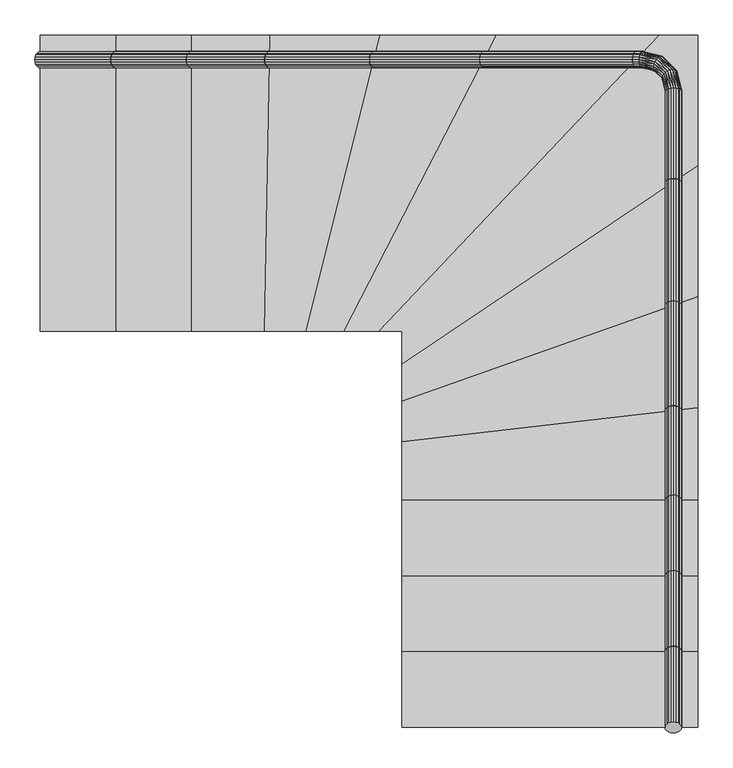
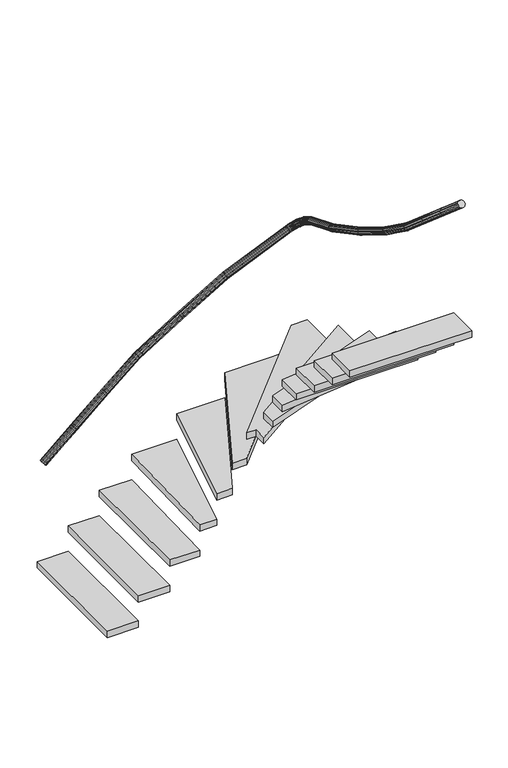
"""IFC4 building model written with IfcOpenShell, lengths in millimetres: stair geometry, 0_3d_modell."""

from ifc_helpers import new_model, si_unit, frame, origin, origin_with_axes, place, context, project, spatial, polyline, outline, extrude, faceted_brep, source, transform, mapped, element, save


def stair_c236abdd(model_context):
    return source(origin(), model_context, "Body", "SolidModel", [
        extrude(outline(polyline([(1049.2205336, 2121.5036957), (1403.2627923, 2121.5036957), (939.4821841, 1221.5036957), (824.5831846, 1221.5036957), (1049.2205336, 2121.5036957)])), frame((0.0, 0.0, 794.2857143), z_axis=(0.0, 0.0, 1.0), x_axis=(1.0, 0.0, 0.0)), (0.0, 0.0, 1.0), 50.0),
        faceted_brep([(1830.8955374, 2022.7272828, 2053.6142572), (1827.811235, 2021.5036957, 2060.987808), (1824.7269327, 2022.7272828, 2068.3613589), (1821.9445433, 2026.2782709, 2075.0131352), (1819.7364266, 2031.8090644, 2080.2920148), (1818.3187285, 2038.7782709, 2083.6812642), (1817.830223, 2046.5036957, 2084.8491199), (1818.3187285, 2054.2291206, 2083.6812642), (1819.7364266, 2061.198327, 2080.2920148), (1821.9445433, 2066.7291206, 2075.0131352), (1824.7269327, 2070.2801086, 2068.3613589), (1827.811235, 2071.5036957, 2060.987808), (1830.8955374, 2070.2801086, 2053.6142572), (1833.6779267, 2066.7291206, 2046.9624808), (1835.8860434, 2061.198327, 2041.6836012), (1837.3037416, 2054.2291206, 2038.2943519), (1837.7922471, 2046.5036957, 2037.1264962), (1837.3037416, 2038.7782709, 2038.2943519), (1835.8860434, 2031.8090644, 2041.6836012), (1833.6779267, 2026.2782709, 2046.9624808), (1918.1254462, 1677.2481385, 2266.8075559), (1916.9018591, 1673.856869, 2259.5592366), (1918.1254462, 1670.4655995, 2252.3109173), (1921.6764343, 1667.4062911, 2245.772114), (1927.2072278, 1664.9784102, 2240.5828904), (1934.1764343, 1663.4196147, 2237.2512037), (1941.9018591, 1662.8824904, 2236.1031827), (1949.627284, 1663.4196147, 2237.2512037), (1956.5964904, 1664.9784102, 2240.5828904), (1962.127284, 1667.4062911, 2245.772114), (1965.678272, 1670.4655995, 2252.3109173), (1966.9018591, 1673.856869, 2259.5592366), (1965.678272, 1677.2481385, 2266.8075559), (1962.127284, 1680.3074469, 2273.3463592), (1956.5964904, 1682.7353278, 2278.5355829), (1949.627284, 1684.2941233, 2281.8672695), (1941.9018591, 1684.8312476, 2283.0152905), (1934.1764343, 1684.2941233, 2281.8672695), (1927.2072278, 1682.7353278, 2278.5355829), (1921.6764343, 1680.3074469, 2273.3463592), (1846.1118218, 2021.5036957, 2068.4537913), (1843.0928107, 2022.7272828, 2075.8539787), (1840.3693214, 2026.2782709, 2082.5297841), (1838.2079481, 2031.8090644, 2087.8277333), (1836.820261, 2038.7782709, 2091.2292261), (1836.3420966, 2046.5036957, 2092.4013006), (1836.820261, 2054.2291206, 2091.2292261), (1838.2079481, 2061.198327, 2087.8277333), (1840.3693214, 2066.7291206, 2082.5297841), (1843.0928107, 2070.2801086, 2075.8539787), (1846.1118218, 2071.5036957, 2068.4537913), (1849.1308329, 2070.2801086, 2061.053604), (1851.8543222, 2066.7291206, 2054.3777985), (1854.0156955, 2061.198327, 2049.0798493), (1855.4033826, 2054.2291206, 2045.6783565), (1855.881547, 2046.5036957, 2044.506282), (1855.4033826, 2038.7782709, 2045.6783565), (1854.0156955, 2031.8090644, 2049.0798493), (1851.8543222, 2026.2782709, 2054.3777985), (1849.1308329, 2022.7272828, 2061.053604), (1884.7017207, 2012.6032946, 2093.9682441), (1881.8914919, 2015.5333905, 2100.9604911), (1880.5298735, 2020.3241085, 2107.2682883), (1880.7501499, 2026.5064996, 2112.2741844), (1882.5307592, 2033.4753883, 2115.4881676), (1885.6974028, 2040.5486112, 2116.5956307), (1889.9401076, 2047.0337921, 2115.4881676), (1894.8435681, 2052.2961161, 2112.2741844), (1899.9277994, 2055.8204705, 2107.2682883), (1904.6951215, 2057.2618667, 2100.9604911), (1908.6788758, 2056.4792109, 2093.9682441), (1911.4891045, 2053.549115, 2086.9759971), (1912.850723, 2048.758397, 2080.6681999), (1912.6304465, 2042.5760059, 2075.6623037), (1910.8498373, 2035.6071172, 2072.4483206), (1907.6831937, 2028.5338943, 2071.3408574), (1903.4404889, 2022.0487134, 2072.4483206), (1898.5370284, 2016.7863894, 2075.6623037), (1893.4527971, 2013.262035, 2080.6681999), (1888.685475, 2011.8206388, 2086.9759971), (1908.001458, 1989.3035573, 2121.0971401), (1907.2188022, 1993.2873116, 2128.0893871), (1908.6601984, 1998.0546337, 2134.3971843), (1912.1845528, 2003.138865, 2139.4030804), (1917.4468768, 2008.0423255, 2142.6170636), (1923.9320577, 2012.2850303, 2143.7245267), (1931.0052806, 2015.4516739, 2142.6170636), (1937.9741693, 2017.2322831, 2139.4030804), (1944.1565604, 2017.4525596, 2134.3971843), (1948.9472784, 2016.0909411, 2128.0893871), (1951.8773743, 2013.2807124, 2121.0971401), (1952.6600301, 2009.2969581, 2114.1048931), (1951.2186339, 2004.529636, 2107.7970959), (1947.6942795, 1999.4454047, 2102.7911997), (1942.4319555, 1994.5419442, 2099.5772166), (1935.9467746, 1990.2992394, 2098.4697534), (1928.8735517, 1987.1325958, 2099.5772166), (1921.904663, 1985.3519865, 2102.7911997), (1915.7222719, 1985.1317101, 2107.7970959), (1910.9315539, 1986.4933285, 2114.1048931), (1916.9018591, 1950.7136584, 2146.6115929), (1918.1254462, 1953.7326696, 2154.0117802), (1921.6764343, 1956.4561588, 2160.6875857), (1927.2072278, 1958.6175321, 2165.9855349), (1934.1764343, 1960.0052192, 2169.3870277), (1941.9018591, 1960.4833836, 2170.5591022), (1949.627284, 1960.0052192, 2169.3870277), (1956.5964904, 1958.6175321, 2165.9855349), (1962.127284, 1956.4561588, 2160.6875857), (1965.678272, 1953.7326696, 2154.0117802), (1966.9018591, 1950.7136584, 2146.6115929), (1965.678272, 1947.6946473, 2139.2114055), (1962.127284, 1944.971158, 2132.5356001), (1956.5964904, 1942.8097847, 2127.2376509), (1949.627284, 1941.4220976, 2123.8361581), (1941.9018591, 1940.9439332, 2122.6640835), (1934.1764343, 1941.4220976, 2123.8361581), (1927.2072278, 1942.8097847, 2127.2376509), (1921.6764343, 1944.971158, 2132.5356001), (1918.1254462, 1947.6946473, 2139.2114055)], [[[0, 1, 2, 3, 4, 5, 6, 7, 8, 9, 10, 11, 12, 13, 14, 15, 16, 17, 18, 19]], [[20, 21, 22, 23, 24, 25, 26, 27, 28, 29, 30, 31, 32, 33, 34, 35, 36, 37, 38, 39]], [[2, 1, 40, 41]], [[3, 2, 41, 42]], [[4, 3, 42, 43]], [[5, 4, 43, 44]], [[6, 5, 44, 45]], [[7, 6, 45, 46]], [[8, 7, 46, 47]], [[9, 8, 47, 48]], [[10, 9, 48, 49]], [[11, 10, 49, 50]], [[12, 11, 50, 51]], [[13, 12, 51, 52]], [[14, 13, 52, 53]], [[15, 14, 53, 54]], [[16, 15, 54, 55]], [[17, 16, 55, 56]], [[18, 17, 56, 57]], [[19, 18, 57, 58]], [[0, 19, 58, 59]], [[1, 0, 59, 40]], [[41, 40, 60]], [[61, 41, 60]], [[42, 41, 61]], [[62, 42, 61]], [[43, 42, 62]], [[63, 43, 62]], [[44, 43, 63]], [[64, 44, 63]], [[45, 44, 64]], [[65, 45, 64]], [[46, 45, 65]], [[66, 46, 65]], [[47, 46, 66]], [[67, 47, 66]], [[48, 47, 67]], [[68, 48, 67]], [[49, 48, 68]], [[69, 49, 68]], [[50, 49, 69]], [[70, 50, 69]], [[51, 50, 70]], [[71, 51, 70]], [[52, 51, 71]], [[72, 52, 71]], [[53, 52, 72]], [[73, 53, 72]], [[54, 53, 73]], [[74, 54, 73]], [[55, 54, 74]], [[75, 55, 74]], [[56, 55, 75]], [[76, 56, 75]], [[57, 56, 76]], [[77, 57, 76]], [[58, 57, 77]], [[78, 58, 77]], [[59, 58, 78]], [[79, 59, 78]], [[40, 59, 79]], [[60, 40, 79]], [[61, 60, 80]], [[81, 61, 80]], [[62, 61, 81]], [[82, 62, 81]], [[63, 62, 82]], [[83, 63, 82]], [[64, 63, 83]], [[84, 64, 83]], [[65, 64, 84]], [[85, 65, 84]], [[66, 65, 85]], [[86, 66, 85]], [[67, 66, 86]], [[87, 67, 86]], [[68, 67, 87]], [[88, 68, 87]], [[69, 68, 88]], [[89, 69, 88]], [[70, 69, 89]], [[90, 70, 89]], [[71, 70, 90]], [[91, 71, 90]], [[72, 71, 91]], [[92, 72, 91]], [[73, 72, 92]], [[93, 73, 92]], [[74, 73, 93]], [[94, 74, 93]], [[75, 74, 94]], [[95, 75, 94]], [[76, 75, 95]], [[96, 76, 95]], [[77, 76, 96]], [[97, 77, 96]], [[78, 77, 97]], [[98, 78, 97]], [[79, 78, 98]], [[99, 79, 98]], [[60, 79, 99]], [[80, 60, 99]], [[81, 80, 100]], [[101, 81, 100]], [[82, 81, 101]], [[102, 82, 101]], [[83, 82, 102]], [[103, 83, 102]], [[84, 83, 103]], [[104, 84, 103]], [[85, 84, 104]], [[105, 85, 104]], [[86, 85, 105]], [[106, 86, 105]], [[87, 86, 106]], [[107, 87, 106]], [[88, 87, 107]], [[108, 88, 107]], [[89, 88, 108]], [[109, 89, 108]], [[90, 89, 109]], [[110, 90, 109]], [[91, 90, 110]], [[111, 91, 110]], [[92, 91, 111]], [[112, 92, 111]], [[93, 92, 112]], [[113, 93, 112]], [[94, 93, 113]], [[114, 94, 113]], [[95, 94, 114]], [[115, 95, 114]], [[96, 95, 115]], [[116, 96, 115]], [[97, 96, 116]], [[117, 97, 116]], [[98, 97, 117]], [[118, 98, 117]], [[99, 98, 118]], [[119, 99, 118]], [[80, 99, 119]], [[100, 80, 119]], [[101, 100, 21, 20]], [[102, 101, 20, 39]], [[103, 102, 39, 38]], [[104, 103, 38, 37]], [[105, 104, 37, 36]], [[106, 105, 36, 35]], [[107, 106, 35, 34]], [[108, 107, 34, 33]], [[109, 108, 33, 32]], [[110, 109, 32, 31]], [[111, 110, 31, 30]], [[112, 111, 30, 29]], [[113, 112, 29, 28]], [[114, 113, 28, 27]], [[115, 114, 27, 26]], [[116, 115, 26, 25]], [[117, 116, 25, 24]], [[118, 117, 24, 23]], [[119, 118, 23, 22]], [[100, 119, 22, 21]]]),
        extrude(outline(polyline([(2016.9018591, 1724.0707938), (2016.9018591, 1326.2140709), (1116.9018591, 1007.5896473), (1116.9018591, 1121.5036957), (2016.9018591, 1724.0707938)])), frame((0.0, 0.0, 1390.0), z_axis=(0.0, 0.0, 1.0), x_axis=(1.0, 0.0, 0.0)), (0.0, 0.0, 1.0), 50.0),
        extrude(outline(polyline([(1.2235871, -7.9923214), (0.0, 0.0), (1.2235871, 7.9923214), (4.7745752, 15.2022986), (10.3053687, 20.924169), (17.2745752, 24.5978359), (25.0, 25.8636953), (32.7254249, 24.5978359), (39.6946313, 20.924169), (45.2254249, 15.2022986), (48.7764129, 7.9923214), (50.0, 0.0), (48.7764129, -7.9923214), (45.2254249, -15.2022986), (39.6946313, -20.9241691), (32.7254249, -24.5978359), (25.0, -25.8636953), (17.2745752, -24.5978359), (10.3053687, -20.9241691), (4.7745752, -15.2022986), (1.2235871, -7.9923214)])), frame((16.9018591, 2021.5036957, 869.5592366), z_axis=(0.756928710285757, 0.0, 0.6534974579484916), x_axis=(0.0, 1.0, 0.0)), (0.0, 0.0, 1.0), 303.8595272),
        extrude(outline(polyline([(246.9018591, 2121.5036957), (476.9018591, 2121.5036957), (476.9018591, 1221.5036957), (246.9018591, 1221.5036957), (246.9018591, 2121.5036957)])), frame((0.0, 0.0, 198.5714286), z_axis=(0.0, 0.0, 1.0), x_axis=(1.0, 0.0, 0.0)), (0.0, 0.0, 1.0), 50.0),
        extrude(outline(polyline([(2016.9018591, 476.9018591), (2016.9018591, 246.9018591), (1116.9018591, 246.9018591), (1116.9018591, 476.9018591), (2016.9018591, 476.9018591)])), frame((0.0, 0.0, 2184.2857143), z_axis=(0.0, 0.0, 1.0), x_axis=(1.0, 0.0, 0.0)), (0.0, 0.0, 1.0), 50.0),
        extrude(outline(polyline([(2016.9018591, 1326.2140709), (2016.9018591, 988.8933271), (1116.9018591, 884.9103911), (1116.9018591, 1007.5896473), (2016.9018591, 1326.2140709)])), frame((0.0, 0.0, 1588.5714286), z_axis=(0.0, 0.0, 1.0), x_axis=(1.0, 0.0, 0.0)), (0.0, 0.0, 1.0), 50.0),
        faceted_brep([(1918.1254462, 1295.6744399, 2451.1987943), (1916.9018591, 1299.6620356, 2458.1306652), (1918.1254462, 1303.6496314, 2465.062536), (1921.6764343, 1307.2468935, 2471.3158671), (1927.2072278, 1310.1016969, 2476.2785387), (1934.1764343, 1311.9345935, 2479.46477), (1941.9018591, 1312.5661666, 2480.5626705), (1949.627284, 1311.9345935, 2479.46477), (1956.5964904, 1310.1016969, 2476.2785387), (1962.127284, 1307.2468935, 2471.3158671), (1965.678272, 1303.6496314, 2465.062536), (1966.9018591, 1299.6620356, 2458.1306652), (1965.678272, 1295.6744399, 2451.1987943), (1962.127284, 1292.0771778, 2444.9454632), (1956.5964904, 1289.2223744, 2439.9827916), (1949.627284, 1287.3894778, 2436.7965603), (1941.9018591, 1286.7579047, 2435.6986598), (1934.1764343, 1287.3894778, 2436.7965603), (1927.2072278, 1289.2223744, 2439.9827916), (1921.6764343, 1292.0771778, 2444.9454632), (1918.1254462, 984.692421, 2663.3376045), (1916.9018591, 980.2280824, 2656.7020937), (1918.1254462, 975.7637439, 2650.066583), (1921.6764343, 971.7364059, 2644.0806023), (1927.2072278, 968.5402924, 2639.3301012), (1934.1764343, 966.4882612, 2636.2800917), (1941.9018591, 965.7811794, 2635.22913), (1949.627284, 966.4882612, 2636.2800917), (1956.5964904, 968.5402924, 2639.3301012), (1962.127284, 971.7364059, 2644.0806023), (1965.678272, 975.7637439, 2650.066583), (1966.9018591, 980.2280824, 2656.7020937), (1965.678272, 984.692421, 2663.3376045), (1962.127284, 988.719759, 2669.3235852), (1956.5964904, 991.9158725, 2674.0740863), (1949.627284, 993.9679037, 2677.1240958), (1941.9018591, 994.6749855, 2678.1750575), (1934.1764343, 993.9679037, 2677.1240958), (1927.2072278, 991.9158725, 2674.0740863), (1921.6764343, 988.719759, 2669.3235852)], [[[0, 1, 2, 3, 4, 5, 6, 7, 8, 9, 10, 11, 12, 13, 14, 15, 16, 17, 18, 19]], [[20, 21, 22, 23, 24, 25, 26, 27, 28, 29, 30, 31, 32, 33, 34, 35, 36, 37, 38, 39]], [[2, 1, 21, 20]], [[3, 2, 20, 39]], [[4, 3, 39, 38]], [[5, 4, 38, 37]], [[6, 5, 37, 36]], [[7, 6, 36, 35]], [[8, 7, 35, 34]], [[9, 8, 34, 33]], [[10, 9, 33, 32]], [[11, 10, 32, 31]], [[12, 11, 31, 30]], [[13, 12, 30, 29]], [[14, 13, 29, 28]], [[15, 14, 28, 27]], [[16, 15, 27, 26]], [[17, 16, 26, 25]], [[18, 17, 25, 24]], [[19, 18, 24, 23]], [[0, 19, 23, 22]], [[1, 0, 22, 21]]]),
        extrude(outline(polyline([(16.9018591, 2121.5036957), (246.9018591, 2121.5036957), (246.9018591, 1221.5036957), (16.9018591, 1221.5036957), (16.9018591, 2121.5036957)])), origin_with_axes(), (0.0, 0.0, 1.0), 50.0),
        faceted_brep([(482.0819027, 2022.7272828, 1260.6154227), (476.9018591, 2021.5036957, 1266.7020937), (471.7218155, 2022.7272828, 1272.7887648), (467.0488307, 2026.2782709, 1278.2796301), (463.340329, 2031.8090644, 1282.6372054), (460.9593243, 2038.7782709, 1285.434941), (460.138886, 2046.5036957, 1286.398975), (460.9593243, 2054.2291206, 1285.434941), (463.340329, 2061.198327, 1282.6372054), (467.0488307, 2066.7291206, 1278.2796301), (471.7218155, 2070.2801086, 1272.7887648), (476.9018591, 2071.5036957, 1266.7020937), (482.0819027, 2070.2801086, 1260.6154227), (486.7548875, 2066.7291206, 1255.1245574), (490.4633893, 2061.198327, 1250.7669821), (492.844394, 2054.2291206, 1247.9692465), (493.6648323, 2046.5036957, 1247.0052125), (492.844394, 2038.7782709, 1247.9692465), (490.4633893, 2031.8090644, 1250.7669821), (486.7548875, 2026.2782709, 1255.1245574), (708.8971261, 2022.7272828, 1471.7522459), (713.6098217, 2021.5036957, 1465.2735223), (718.3225173, 2022.7272828, 1458.7947987), (722.5739015, 2026.2782709, 1452.9502578), (725.947819, 2031.8090644, 1448.3120038), (728.1140074, 2038.7782709, 1445.3340614), (728.8604251, 2046.5036957, 1444.3079324), (728.1140074, 2054.2291206, 1445.3340614), (725.947819, 2061.198327, 1448.3120038), (722.5739015, 2066.7291206, 1452.9502578), (718.3225173, 2070.2801086, 1458.7947987), (713.6098217, 2071.5036957, 1465.2735223), (708.8971261, 2070.2801086, 1471.7522459), (704.645742, 2066.7291206, 1477.5967869), (701.2718245, 2061.198327, 1482.2350408), (699.1056361, 2054.2291206, 1485.2129832), (698.3592184, 2046.5036957, 1486.2391122), (699.1056361, 2038.7782709, 1485.2129832), (701.2718245, 2031.8090644, 1482.2350408), (704.645742, 2026.2782709, 1477.5967869)], [[[0, 1, 2, 3, 4, 5, 6, 7, 8, 9, 10, 11, 12, 13, 14, 15, 16, 17, 18, 19]], [[20, 21, 22, 23, 24, 25, 26, 27, 28, 29, 30, 31, 32, 33, 34, 35, 36, 37, 38, 39]], [[2, 1, 21, 20]], [[3, 2, 20, 39]], [[4, 3, 39, 38]], [[5, 4, 38, 37]], [[6, 5, 37, 36]], [[7, 6, 36, 35]], [[8, 7, 35, 34]], [[9, 8, 34, 33]], [[10, 9, 33, 32]], [[11, 10, 32, 31]], [[12, 11, 31, 30]], [[13, 12, 30, 29]], [[14, 13, 29, 28]], [[15, 14, 28, 27]], [[16, 15, 27, 26]], [[17, 16, 26, 25]], [[18, 17, 25, 24]], [[19, 18, 24, 23]], [[0, 19, 23, 22]], [[1, 0, 22, 21]]]),
        extrude(outline(polyline([(1403.2627923, 2121.5036957), (1898.8029965, 2121.5036957), (1046.9018591, 1221.5036957), (939.4821841, 1221.5036957), (1403.2627923, 2121.5036957)])), frame((0.0, 0.0, 992.8571429), z_axis=(0.0, 0.0, 1.0), x_axis=(1.0, 0.0, 0.0)), (0.0, 0.0, 1.0), 50.0),
        extrude(outline(polyline([(2016.9018591, 246.9018591), (2016.9018591, 16.9018591), (1116.9018591, 16.9018591), (1116.9018591, 246.9018591), (2016.9018591, 246.9018591)])), frame((0.0, 0.0, 2382.8571429), z_axis=(0.0, 0.0, 1.0), x_axis=(1.0, 0.0, 0.0)), (0.0, 0.0, 1.0), 50.0),
        faceted_brep([(252.1248208, 2022.7272828, 1062.0810477), (246.9018591, 2021.5036957, 1068.1306652), (241.6788974, 2022.7272828, 1074.1802827), (236.9671956, 2026.2782709, 1079.6377215), (233.2279679, 2031.8090644, 1083.9687694), (230.8272359, 2038.7782709, 1086.7494734), (230.0, 2046.5036957, 1087.7076387), (230.8272359, 2054.2291206, 1086.7494734), (233.2279679, 2061.198327, 1083.9687694), (236.9671956, 2066.7291206, 1079.6377215), (241.6788974, 2070.2801086, 1074.1802827), (246.9018591, 2071.5036957, 1068.1306652), (252.1248208, 2070.2801086, 1062.0810477), (256.8365226, 2066.7291206, 1056.6236089), (260.5757504, 2061.198327, 1052.2925609), (262.9764824, 2054.2291206, 1049.511857), (263.8037182, 2046.5036957, 1048.5536917), (262.9764824, 2038.7782709, 1049.511857), (260.5757504, 2031.8090644, 1052.2925609), (256.8365226, 2026.2782709, 1056.6236089), (471.7218155, 2022.7272828, 1272.7887648), (476.9018591, 2021.5036957, 1266.7020937), (482.0819027, 2022.7272828, 1260.6154227), (486.7548875, 2026.2782709, 1255.1245574), (490.4633893, 2031.8090644, 1250.7669821), (492.844394, 2038.7782709, 1247.9692465), (493.6648323, 2046.5036957, 1247.0052125), (492.844394, 2054.2291206, 1247.9692465), (490.4633893, 2061.198327, 1250.7669821), (486.7548875, 2066.7291206, 1255.1245574), (482.0819027, 2070.2801086, 1260.6154227), (476.9018591, 2071.5036957, 1266.7020937), (471.7218155, 2070.2801086, 1272.7887648), (467.0488307, 2066.7291206, 1278.2796301), (463.340329, 2061.198327, 1282.6372054), (460.9593243, 2054.2291206, 1285.434941), (460.138886, 2046.5036957, 1286.398975), (460.9593243, 2038.7782709, 1285.434941), (463.340329, 2031.8090644, 1282.6372054), (467.0488307, 2026.2782709, 1278.2796301)], [[[0, 1, 2, 3, 4, 5, 6, 7, 8, 9, 10, 11, 12, 13, 14, 15, 16, 17, 18, 19]], [[20, 21, 22, 23, 24, 25, 26, 27, 28, 29, 30, 31, 32, 33, 34, 35, 36, 37, 38, 39]], [[2, 1, 21, 20]], [[3, 2, 20, 39]], [[4, 3, 39, 38]], [[5, 4, 38, 37]], [[6, 5, 37, 36]], [[7, 6, 36, 35]], [[8, 7, 35, 34]], [[9, 8, 34, 33]], [[10, 9, 33, 32]], [[11, 10, 32, 31]], [[12, 11, 31, 30]], [[13, 12, 30, 29]], [[14, 13, 29, 28]], [[15, 14, 28, 27]], [[16, 15, 27, 26]], [[17, 16, 26, 25]], [[18, 17, 25, 24]], [[19, 18, 24, 23]], [[0, 19, 23, 22]], [[1, 0, 22, 21]]]),
        extrude(outline(polyline([(2016.9018591, 706.9018591), (2016.9018591, 476.9018591), (1116.9018591, 476.9018591), (1116.9018591, 706.9018591), (2016.9018591, 706.9018591)])), frame((0.0, 0.0, 1985.7142857), z_axis=(0.0, 0.0, 1.0), x_axis=(1.0, 0.0, 0.0)), (0.0, 0.0, 1.0), 50.0),
        extrude(outline(polyline([(1898.8029965, 2121.5036957), (2016.9018591, 2121.5036957), (2016.9018591, 1724.0707938), (1116.9018591, 1121.5036957), (1116.9018591, 1221.5036957), (1046.9018591, 1221.5036957), (1898.8029965, 2121.5036957)])), frame((0.0, 0.0, 1191.4285714), z_axis=(0.0, 0.0, 1.0), x_axis=(1.0, 0.0, 0.0)), (0.0, 0.0, 1.0), 50.0),
        extrude(outline(polyline([(1.2235871, -7.9923214), (0.0, 0.0), (1.2235871, 7.9923214), (4.7745752, 15.2022986), (10.3053687, 20.9241691), (17.2745752, 24.5978359), (25.0, 25.8636953), (32.7254249, 24.5978359), (39.6946313, 20.9241691), (45.2254249, 15.2022986), (48.7764129, 7.9923214), (50.0, 0.0), (48.7764129, -7.9923214), (45.2254249, -15.2022986), (39.6946313, -20.924169), (32.7254249, -24.5978359), (25.0, -25.8636953), (17.2745752, -24.5978359), (10.3053687, -20.924169), (4.7745752, -15.2022986), (1.2235871, -7.9923214)])), frame((1916.9018591, 476.9018591, 3053.8449509), z_axis=(0.0, -0.7569287102856931, 0.6534974579485656), x_axis=(1.0, 0.0, 0.0)), (0.0, 0.0, 1.0), 303.8595272),
        faceted_brep([(1918.1254462, 701.932844, 2849.004659), (1916.9018591, 706.9018591, 2855.2735223), (1918.1254462, 711.8708742, 2861.5423857), (1921.6764343, 716.3534875, 2867.197609), (1927.2072278, 719.9109095, 2871.6856196), (1934.1764343, 722.194915, 2874.5670998), (1941.9018591, 722.9819297, 2875.5599903), (1949.627284, 722.194915, 2874.5670998), (1956.5964904, 719.9109095, 2871.6856196), (1962.127284, 716.3534875, 2867.197609), (1965.678272, 711.8708742, 2861.5423857), (1966.9018591, 706.9018591, 2855.2735223), (1965.678272, 701.932844, 2849.004659), (1962.127284, 697.4502308, 2843.3494356), (1956.5964904, 693.8928087, 2838.861425), (1949.627284, 691.6088032, 2835.9799448), (1941.9018591, 690.8217885, 2834.9870544), (1934.1764343, 691.6088032, 2835.9799448), (1927.2072278, 693.8928087, 2838.861425), (1921.6764343, 697.4502308, 2843.3494356), (1918.1254462, 482.1248208, 3059.8945684), (1916.9018591, 476.9018591, 3053.8449509), (1918.1254462, 471.6788974, 3047.7953334), (1921.6764343, 466.9671956, 3042.3378946), (1927.2072278, 463.2279679, 3038.0068466), (1934.1764343, 460.8272359, 3035.2261427), (1941.9018591, 460.0, 3034.2679774), (1949.627284, 460.8272359, 3035.2261427), (1956.5964904, 463.2279679, 3038.0068466), (1962.127284, 466.9671956, 3042.3378946), (1965.678272, 471.6788974, 3047.7953334), (1966.9018591, 476.9018591, 3053.8449509), (1965.678272, 482.1248208, 3059.8945684), (1962.127284, 486.8365226, 3065.3520072), (1956.5964904, 490.5757504, 3069.6830552), (1949.627284, 492.9764824, 3072.4637591), (1941.9018591, 493.8037182, 3073.4219244), (1934.1764343, 492.9764824, 3072.4637591), (1927.2072278, 490.5757504, 3069.6830552), (1921.6764343, 486.8365226, 3065.3520072)], [[[0, 1, 2, 3, 4, 5, 6, 7, 8, 9, 10, 11, 12, 13, 14, 15, 16, 17, 18, 19]], [[20, 21, 22, 23, 24, 25, 26, 27, 28, 29, 30, 31, 32, 33, 34, 35, 36, 37, 38, 39]], [[2, 1, 21, 20]], [[3, 2, 20, 39]], [[4, 3, 39, 38]], [[5, 4, 38, 37]], [[6, 5, 37, 36]], [[7, 6, 36, 35]], [[8, 7, 35, 34]], [[9, 8, 34, 33]], [[10, 9, 33, 32]], [[11, 10, 32, 31]], [[12, 11, 31, 30]], [[13, 12, 30, 29]], [[14, 13, 29, 28]], [[15, 14, 28, 27]], [[16, 15, 27, 26]], [[17, 16, 26, 25]], [[18, 17, 25, 24]], [[19, 18, 24, 23]], [[0, 19, 23, 22]], [[1, 0, 22, 21]]]),
        faceted_brep([(1368.2462303, 2022.7272828, 1855.277549), (1364.6144083, 2021.5036957, 1862.4163795), (1360.9825862, 2022.7272828, 1869.5552099), (1357.7062723, 2026.2782709, 1875.9952419), (1355.1061748, 2031.8090644, 1881.1060802), (1353.4368094, 2038.7782709, 1884.3874404), (1352.8615853, 2046.5036957, 1885.51812), (1353.4368094, 2054.2291206, 1884.3874404), (1355.1061748, 2061.198327, 1881.1060802), (1357.7062723, 2066.7291206, 1875.9952419), (1360.9825862, 2070.2801086, 1869.5552099), (1364.6144083, 2071.5036957, 1862.4163795), (1368.2462303, 2070.2801086, 1855.277549), (1371.5225443, 2066.7291206, 1848.8375171), (1374.1226418, 2061.198327, 1843.7266788), (1375.7920071, 2054.2291206, 1840.4453186), (1376.3672312, 2046.5036957, 1839.3146389), (1375.7920071, 2038.7782709, 1840.4453186), (1374.1226418, 2031.8090644, 1843.7266788), (1371.5225443, 2026.2782709, 1848.8375171), (1824.7269327, 2022.7272828, 2068.3613589), (1827.811235, 2021.5036957, 2060.987808), (1830.8955374, 2022.7272828, 2053.6142572), (1833.6779267, 2026.2782709, 2046.9624808), (1835.8860434, 2031.8090644, 2041.6836012), (1837.3037416, 2038.7782709, 2038.2943519), (1837.7922471, 2046.5036957, 2037.1264962), (1837.3037416, 2054.2291206, 2038.2943519), (1835.8860434, 2061.198327, 2041.6836012), (1833.6779267, 2066.7291206, 2046.9624808), (1830.8955374, 2070.2801086, 2053.6142572), (1827.811235, 2071.5036957, 2060.987808), (1824.7269327, 2070.2801086, 2068.3613589), (1821.9445433, 2066.7291206, 2075.0131352), (1819.7364266, 2061.198327, 2080.2920148), (1818.3187285, 2054.2291206, 2083.6812642), (1817.830223, 2046.5036957, 2084.8491199), (1818.3187285, 2038.7782709, 2083.6812642), (1819.7364266, 2031.8090644, 2080.2920148), (1821.9445433, 2026.2782709, 2075.0131352)], [[[0, 1, 2, 3, 4, 5, 6, 7, 8, 9, 10, 11, 12, 13, 14, 15, 16, 17, 18, 19]], [[20, 21, 22, 23, 24, 25, 26, 27, 28, 29, 30, 31, 32, 33, 34, 35, 36, 37, 38, 39]], [[2, 1, 21, 20]], [[3, 2, 20, 39]], [[4, 3, 39, 38]], [[5, 4, 38, 37]], [[6, 5, 37, 36]], [[7, 6, 36, 35]], [[8, 7, 35, 34]], [[9, 8, 34, 33]], [[10, 9, 33, 32]], [[11, 10, 32, 31]], [[12, 11, 31, 30]], [[13, 12, 30, 29]], [[14, 13, 29, 28]], [[15, 14, 28, 27]], [[16, 15, 27, 26]], [[17, 16, 26, 25]], [[18, 17, 25, 24]], [[19, 18, 24, 23]], [[0, 19, 23, 22]], [[1, 0, 22, 21]]]),
        faceted_brep([(718.3225173, 2022.7272828, 1458.7947987), (713.6098217, 2021.5036957, 1465.2735223), (708.8971261, 2022.7272828, 1471.7522459), (704.645742, 2026.2782709, 1477.5967869), (701.2718245, 2031.8090644, 1482.2350408), (699.1056361, 2038.7782709, 1485.2129832), (698.3592184, 2046.5036957, 1486.2391122), (699.1056361, 2054.2291206, 1485.2129832), (701.2718245, 2061.198327, 1482.2350408), (704.645742, 2066.7291206, 1477.5967869), (708.8971261, 2070.2801086, 1471.7522459), (713.6098217, 2071.5036957, 1465.2735223), (718.3225173, 2070.2801086, 1458.7947987), (722.5739015, 2066.7291206, 1452.9502578), (725.947819, 2061.198327, 1448.3120038), (728.1140074, 2054.2291206, 1445.3340614), (728.8604251, 2046.5036957, 1444.3079324), (728.1140074, 2038.7782709, 1445.3340614), (725.947819, 2031.8090644, 1448.3120038), (722.5739015, 2026.2782709, 1452.9502578), (1026.3366143, 2022.7272828, 1670.6674124), (1030.5007545, 2021.5036957, 1663.8449509), (1034.6648948, 2022.7272828, 1657.0224894), (1038.42142, 2026.2782709, 1650.867858), (1041.4026152, 2031.8090644, 1645.9835149), (1043.3166604, 2038.7782709, 1642.8475735), (1043.9761954, 2046.5036957, 1641.7670018), (1043.3166604, 2054.2291206, 1642.8475735), (1041.4026152, 2061.198327, 1645.9835149), (1038.42142, 2066.7291206, 1650.867858), (1034.6648948, 2070.2801086, 1657.0224894), (1030.5007545, 2071.5036957, 1663.8449509), (1026.3366143, 2070.2801086, 1670.6674124), (1022.5800891, 2066.7291206, 1676.8220438), (1019.5988939, 2061.198327, 1681.7063869), (1017.6848487, 2054.2291206, 1684.8423282), (1017.0253137, 2046.5036957, 1685.9229), (1017.6848487, 2038.7782709, 1684.8423282), (1019.5988939, 2031.8090644, 1681.7063869), (1022.5800891, 2026.2782709, 1676.8220438)], [[[0, 1, 2, 3, 4, 5, 6, 7, 8, 9, 10, 11, 12, 13, 14, 15, 16, 17, 18, 19]], [[20, 21, 22, 23, 24, 25, 26, 27, 28, 29, 30, 31, 32, 33, 34, 35, 36, 37, 38, 39]], [[2, 1, 21, 20]], [[3, 2, 20, 39]], [[4, 3, 39, 38]], [[5, 4, 38, 37]], [[6, 5, 37, 36]], [[7, 6, 36, 35]], [[8, 7, 35, 34]], [[9, 8, 34, 33]], [[10, 9, 33, 32]], [[11, 10, 32, 31]], [[12, 11, 31, 30]], [[13, 12, 30, 29]], [[14, 13, 29, 28]], [[15, 14, 28, 27]], [[16, 15, 27, 26]], [[17, 16, 26, 25]], [[18, 17, 25, 24]], [[19, 18, 24, 23]], [[0, 19, 23, 22]], [[1, 0, 22, 21]]]),
        extrude(outline(polyline([(476.9018591, 2121.5036957), (714.9514143, 2121.5036957), (698.852304, 1221.5036957), (476.9018591, 1221.5036957), (476.9018591, 2121.5036957)])), frame((0.0, 0.0, 397.1428571), z_axis=(0.0, 0.0, 1.0), x_axis=(1.0, 0.0, 0.0)), (0.0, 0.0, 1.0), 50.0),
        extrude(outline(polyline([(2016.9018591, 988.8933271), (2016.9018591, 706.9018591), (1116.9018591, 706.9018591), (1116.9018591, 884.9103911), (2016.9018591, 988.8933271)])), frame((0.0, 0.0, 1787.1428571), z_axis=(0.0, 0.0, 1.0), x_axis=(1.0, 0.0, 0.0)), (0.0, 0.0, 1.0), 50.0),
        faceted_brep([(1034.6648948, 2022.7272828, 1657.0224894), (1030.5007545, 2021.5036957, 1663.8449509), (1026.3366143, 2022.7272828, 1670.6674124), (1022.5800891, 2026.2782709, 1676.8220438), (1019.5988939, 2031.8090644, 1681.7063869), (1017.6848487, 2038.7782709, 1684.8423282), (1017.0253137, 2046.5036957, 1685.9229), (1017.6848487, 2054.2291206, 1684.8423282), (1019.5988939, 2061.198327, 1681.7063869), (1022.5800891, 2066.7291206, 1676.8220438), (1026.3366143, 2070.2801086, 1670.6674124), (1030.5007545, 2071.5036957, 1663.8449509), (1034.6648948, 2070.2801086, 1657.0224894), (1038.42142, 2066.7291206, 1650.867858), (1041.4026152, 2061.198327, 1645.9835149), (1043.3166604, 2054.2291206, 1642.8475735), (1043.9761954, 2046.5036957, 1641.7670018), (1043.3166604, 2038.7782709, 1642.8475735), (1041.4026152, 2031.8090644, 1645.9835149), (1038.42142, 2026.2782709, 1650.867858), (1360.9825862, 2022.7272828, 1869.5552099), (1364.6144083, 2021.5036957, 1862.4163795), (1368.2462303, 2022.7272828, 1855.277549), (1371.5225443, 2026.2782709, 1848.8375171), (1374.1226418, 2031.8090644, 1843.7266788), (1375.7920071, 2038.7782709, 1840.4453186), (1376.3672312, 2046.5036957, 1839.3146389), (1375.7920071, 2054.2291206, 1840.4453186), (1374.1226418, 2061.198327, 1843.7266788), (1371.5225443, 2066.7291206, 1848.8375171), (1368.2462303, 2070.2801086, 1855.277549), (1364.6144083, 2071.5036957, 1862.4163795), (1360.9825862, 2070.2801086, 1869.5552099), (1357.7062723, 2066.7291206, 1875.9952419), (1355.1061748, 2061.198327, 1881.1060802), (1353.4368094, 2054.2291206, 1884.3874404), (1352.8615853, 2046.5036957, 1885.51812), (1353.4368094, 2038.7782709, 1884.3874404), (1355.1061748, 2031.8090644, 1881.1060802), (1357.7062723, 2026.2782709, 1875.9952419)], [[[0, 1, 2, 3, 4, 5, 6, 7, 8, 9, 10, 11, 12, 13, 14, 15, 16, 17, 18, 19]], [[20, 21, 22, 23, 24, 25, 26, 27, 28, 29, 30, 31, 32, 33, 34, 35, 36, 37, 38, 39]], [[2, 1, 21, 20]], [[3, 2, 20, 39]], [[4, 3, 39, 38]], [[5, 4, 38, 37]], [[6, 5, 37, 36]], [[7, 6, 36, 35]], [[8, 7, 35, 34]], [[9, 8, 34, 33]], [[10, 9, 33, 32]], [[11, 10, 32, 31]], [[12, 11, 31, 30]], [[13, 12, 30, 29]], [[14, 13, 29, 28]], [[15, 14, 28, 27]], [[16, 15, 27, 26]], [[17, 16, 26, 25]], [[18, 17, 25, 24]], [[19, 18, 24, 23]], [[0, 19, 23, 22]], [[1, 0, 22, 21]]]),
        faceted_brep([(1918.1254462, 975.7637439, 2650.066583), (1916.9018591, 980.2280824, 2656.7020937), (1918.1254462, 984.692421, 2663.3376045), (1921.6764343, 988.719759, 2669.3235852), (1927.2072278, 991.9158725, 2674.0740863), (1934.1764343, 993.9679037, 2677.1240958), (1941.9018591, 994.6749855, 2678.1750575), (1949.627284, 993.9679037, 2677.1240958), (1956.5964904, 991.9158725, 2674.0740863), (1962.127284, 988.719759, 2669.3235852), (1965.678272, 984.692421, 2663.3376045), (1966.9018591, 980.2280824, 2656.7020937), (1965.678272, 975.7637439, 2650.066583), (1962.127284, 971.7364059, 2644.0806023), (1956.5964904, 968.5402924, 2639.3301012), (1949.627284, 966.4882612, 2636.2800917), (1941.9018591, 965.7811794, 2635.22913), (1934.1764343, 966.4882612, 2636.2800917), (1927.2072278, 968.5402924, 2639.3301012), (1921.6764343, 971.7364059, 2644.0806023), (1918.1254462, 711.8708742, 2861.5423857), (1916.9018591, 706.9018591, 2855.2735223), (1918.1254462, 701.932844, 2849.004659), (1921.6764343, 697.4502308, 2843.3494356), (1927.2072278, 693.8928087, 2838.861425), (1934.1764343, 691.6088032, 2835.9799448), (1941.9018591, 690.8217885, 2834.9870544), (1949.627284, 691.6088032, 2835.9799448), (1956.5964904, 693.8928087, 2838.861425), (1962.127284, 697.4502308, 2843.3494356), (1965.678272, 701.932844, 2849.004659), (1966.9018591, 706.9018591, 2855.2735223), (1965.678272, 711.8708742, 2861.5423857), (1962.127284, 716.3534875, 2867.197609), (1956.5964904, 719.9109095, 2871.6856196), (1949.627284, 722.194915, 2874.5670998), (1941.9018591, 722.9819297, 2875.5599903), (1934.1764343, 722.194915, 2874.5670998), (1927.2072278, 719.9109095, 2871.6856196), (1921.6764343, 716.3534875, 2867.197609)], [[[0, 1, 2, 3, 4, 5, 6, 7, 8, 9, 10, 11, 12, 13, 14, 15, 16, 17, 18, 19]], [[20, 21, 22, 23, 24, 25, 26, 27, 28, 29, 30, 31, 32, 33, 34, 35, 36, 37, 38, 39]], [[2, 1, 21, 20]], [[3, 2, 20, 39]], [[4, 3, 39, 38]], [[5, 4, 38, 37]], [[6, 5, 37, 36]], [[7, 6, 36, 35]], [[8, 7, 35, 34]], [[9, 8, 34, 33]], [[10, 9, 33, 32]], [[11, 10, 32, 31]], [[12, 11, 31, 30]], [[13, 12, 30, 29]], [[14, 13, 29, 28]], [[15, 14, 28, 27]], [[16, 15, 27, 26]], [[17, 16, 26, 25]], [[18, 17, 25, 24]], [[19, 18, 24, 23]], [[0, 19, 23, 22]], [[1, 0, 22, 21]]]),
        extrude(outline(polyline([(714.9514143, 2121.5036957), (1049.2205336, 2121.5036957), (824.5831846, 1221.5036957), (698.852304, 1221.5036957), (714.9514143, 2121.5036957)])), frame((0.0, 0.0, 595.7142857), z_axis=(0.0, 0.0, 1.0), x_axis=(1.0, 0.0, 0.0)), (0.0, 0.0, 1.0), 50.0),
        extrude(outline(polyline([(1.2235871, -7.9923214), (0.0, 0.0), (1.2235871, 7.9923214), (4.7745752, 15.2022986), (10.3053687, 20.924169), (17.2745752, 24.5978359), (25.0, 25.8636953), (32.7254249, 24.5978359), (39.6946313, 20.924169), (45.2254249, 15.2022986), (48.7764129, 7.9923214), (50.0, 0.0), (48.7764129, -7.9923214), (45.2254249, -15.2022986), (39.6946313, -20.924169), (32.7254249, -24.597836), (25.0, -25.8636953), (17.2745752, -24.597836), (10.3053687, -20.924169), (4.7745752, -15.2022986), (1.2235871, -7.9923214)])), frame((1916.9018591, 246.9018591, 3252.4163795), z_axis=(0.0, -0.7569287102857004, 0.6534974579485573), x_axis=(1.0, 0.0, 0.0)), (0.0, 0.0, 1.0), 303.8595272),
        faceted_brep([(1918.1254462, 1670.4655995, 2252.3109173), (1916.9018591, 1673.856869, 2259.5592366), (1918.1254462, 1677.2481385, 2266.8075559), (1921.6764343, 1680.3074469, 2273.3463592), (1927.2072278, 1682.7353278, 2278.5355829), (1934.1764343, 1684.2941233, 2281.8672695), (1941.9018591, 1684.8312476, 2283.0152905), (1949.627284, 1684.2941233, 2281.8672695), (1956.5964904, 1682.7353278, 2278.5355829), (1962.127284, 1680.3074469, 2273.3463592), (1965.678272, 1677.2481385, 2266.8075559), (1966.9018591, 1673.856869, 2259.5592366), (1965.678272, 1670.4655995, 2252.3109173), (1962.127284, 1667.4062911, 2245.772114), (1956.5964904, 1664.9784102, 2240.5828904), (1949.627284, 1663.4196147, 2237.2512037), (1941.9018591, 1662.8824904, 2236.1031827), (1934.1764343, 1663.4196147, 2237.2512037), (1927.2072278, 1664.9784102, 2240.5828904), (1921.6764343, 1667.4062911, 2245.772114), (1918.1254462, 1303.6496314, 2465.062536), (1916.9018591, 1299.6620356, 2458.1306652), (1918.1254462, 1295.6744399, 2451.1987943), (1921.6764343, 1292.0771778, 2444.9454632), (1927.2072278, 1289.2223744, 2439.9827916), (1934.1764343, 1287.3894778, 2436.7965603), (1941.9018591, 1286.7579047, 2435.6986598), (1949.627284, 1287.3894778, 2436.7965603), (1956.5964904, 1289.2223744, 2439.9827916), (1962.127284, 1292.0771778, 2444.9454632), (1965.678272, 1295.6744399, 2451.1987943), (1966.9018591, 1299.6620356, 2458.1306652), (1965.678272, 1303.6496314, 2465.062536), (1962.127284, 1307.2468935, 2471.3158671), (1956.5964904, 1310.1016969, 2476.2785387), (1949.627284, 1311.9345935, 2479.46477), (1941.9018591, 1312.5661666, 2480.5626705), (1934.1764343, 1311.9345935, 2479.46477), (1927.2072278, 1310.1016969, 2476.2785387), (1921.6764343, 1307.2468935, 2471.3158671)], [[[0, 1, 2, 3, 4, 5, 6, 7, 8, 9, 10, 11, 12, 13, 14, 15, 16, 17, 18, 19]], [[20, 21, 22, 23, 24, 25, 26, 27, 28, 29, 30, 31, 32, 33, 34, 35, 36, 37, 38, 39]], [[2, 1, 21, 20]], [[3, 2, 20, 39]], [[4, 3, 39, 38]], [[5, 4, 38, 37]], [[6, 5, 37, 36]], [[7, 6, 36, 35]], [[8, 7, 35, 34]], [[9, 8, 34, 33]], [[10, 9, 33, 32]], [[11, 10, 32, 31]], [[12, 11, 31, 30]], [[13, 12, 30, 29]], [[14, 13, 29, 28]], [[15, 14, 28, 27]], [[16, 15, 27, 26]], [[17, 16, 26, 25]], [[18, 17, 25, 24]], [[19, 18, 24, 23]], [[0, 19, 23, 22]], [[1, 0, 22, 21]]]),
    ])


if __name__ == "__main__":
    model = new_model("IFC4")
    model_context = context("Model", 3, world=origin())
    ifc_project = project(units=[si_unit("LENGTHUNIT", "METRE", prefix="MILLI")], contexts=[model_context])
    site = spatial("IfcSite", under=ifc_project)
    building = spatial("IfcBuilding", under=site)
    placement = place(None, origin())
    stair_shape = stair_c236abdd(model_context)
    element("IfcStair", 1, ObjectType="0_3d_modell", at=placement, inside=building, context=model_context, shape_type="MappedRepresentation", body=[
        mapped(stair_shape, transform((0.0, 0.0, 0.0), x_axis=(1.0, 0.0, 0.0), y_axis=(0.0, 1.0, 0.0), z_axis=(0.0, 0.0, 1.0))),
    ])
    save(model, "model.ifc")

# Revit data of these elements
# Element 1 (IfcStair, "0_3d_modell")
#   Materials on its faces: "*1", "weiss"
# Materials
#   "*1": class "Unassigned", colour RGB 175 175 175, transparency 0
#   "weiss": class "Unassigned", colour RGB 255 255 255, transparency 0
